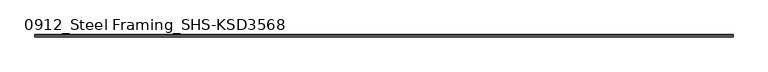
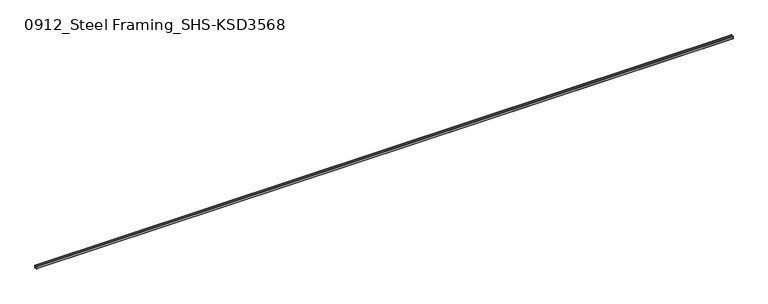
"""IFC4 building model written with IfcOpenShell, lengths in millimetres: beam geometry, 0912_Steel Framing_SHS-KSD3568 : H_SB_ASB_SHS-150x150x6."""

from ifc_helpers import new_model, si_unit, point, frame, frame_2d, origin, place, context, project, spatial, polyline, circle_curve, trimmed, segment, composite_curve, outline, extrude, source, transform, mapped, element, save


def beam_0912_steel_framing_shs_ksd3568_1b1479d8(model_context):
    return source(origin(), model_context, "Body", "SweptSolid", [
        extrude(outline(composite_curve([segment(polyline([(75.0, 63.0), (75.0, -63.0)]), True, "CONTINUOUS"), segment(trimmed(circle_curve(frame_2d((63.0, -63.0)), 12.0), [point((75.0, -63.0))], [point((63.0, -75.0))], False, "CARTESIAN"), True, "CONTINUOUS"), segment(polyline([(63.0, -75.0), (-63.0, -75.0)]), True, "CONTINUOUS"), segment(trimmed(circle_curve(frame_2d((-63.0, -63.0)), 12.0), [point((-63.0, -75.0))], [point((-75.0, -63.0))], False, "CARTESIAN"), True, "CONTINUOUS"), segment(polyline([(-75.0, -63.0), (-75.0, 63.0)]), True, "CONTINUOUS"), segment(trimmed(circle_curve(frame_2d((-63.0, 63.0)), 12.0), [point((-75.0, 63.0))], [point((-63.0, 75.0))], False, "CARTESIAN"), True, "CONTINUOUS"), segment(polyline([(-63.0, 75.0), (63.0, 75.0)]), True, "CONTINUOUS"), segment(trimmed(circle_curve(frame_2d((63.0, 63.0)), 12.0), [point((63.0, 75.0))], [point((75.0, 63.0))], False, "CARTESIAN"), True, "CONTINUOUS")], self_intersect=False), holes=[composite_curve([segment(trimmed(circle_curve(frame_2d((-63.0, 63.0)), 6.0), [point((-63.0, 69.0))], [point((-69.0, 63.0))], True, "CARTESIAN"), True, "CONTINUOUS"), segment(polyline([(-69.0, 63.0), (-69.0, -63.0)]), True, "CONTINUOUS"), segment(trimmed(circle_curve(frame_2d((-63.0, -63.0)), 6.0), [point((-69.0, -63.0))], [point((-63.0, -69.0))], True, "CARTESIAN"), True, "CONTINUOUS"), segment(polyline([(-63.0, -69.0), (63.0, -69.0)]), True, "CONTINUOUS"), segment(trimmed(circle_curve(frame_2d((63.0, -63.0)), 6.0), [point((63.0, -69.0))], [point((69.0, -63.0))], True, "CARTESIAN"), True, "CONTINUOUS"), segment(polyline([(69.0, -63.0), (69.0, 63.0)]), True, "CONTINUOUS"), segment(trimmed(circle_curve(frame_2d((63.0, 63.0)), 6.0), [point((69.0, 63.0))], [point((63.0, 69.0))], True, "CARTESIAN"), True, "CONTINUOUS"), segment(polyline([(63.0, 69.0), (-63.0, 69.0)]), True, "CONTINUOUS")], self_intersect=False)]), frame((-20590.0, 0.0, 0.0), z_axis=(1.0, 0.0, 0.0), x_axis=(0.0, 1.0, 0.0)), (0.0, 0.0, 1.0), 41180.0),
    ])


if __name__ == "__main__":
    model = new_model("IFC4")
    model_context = context("Model", 3, world=origin())
    ifc_project = project(units=[si_unit("LENGTHUNIT", "METRE", prefix="MILLI")], contexts=[model_context])
    site = spatial("IfcSite", under=ifc_project)
    building = spatial("IfcBuilding", under=site)
    placement = place(None, origin())
    beam_0912_steel_framing_shs_ksd3568_shape = beam_0912_steel_framing_shs_ksd3568_1b1479d8(model_context)
    element("IfcBeam", 1, ObjectType="0912_Steel Framing_SHS-KSD3568 : H_SB_ASB_SHS-150x150x6", at=placement, inside=building, context=model_context, shape_type="MappedRepresentation", body=[
        mapped(beam_0912_steel_framing_shs_ksd3568_shape, transform((0.0, 0.0, 0.0), x_axis=(1.0, 0.0, 0.0), y_axis=(0.0, 1.0, 0.0), z_axis=(0.0, 0.0, 1.0))),
    ])
    save(model, "model.ifc")

# Revit data of these elements
# Type "0912_Steel Framing_SHS-KSD3568 : H_SB_ASB_SHS-150x150x6"
#   H_WM Code_1 = "S01AA002-00001 | Main Steel Structure Fabrication Work | Shelter/Building | Medium Steel - Standard (90KG/M>Weight≥30KG/M) | Material: (   )"
#   H_WM Code_2 = "S03AA028-00001 | Main Steel Structure Erection Work | Shelter/Building | Medium Steel (90KG/M>Weight≥30KG/M) | Material: (   )"
#   H_WM Code_3 = "S01AA010-00001 | Main Steel Structure Fabrication Work | Shelter/Building | Steel Painting/Coating | for Non-Fireproofed Steel Surface, Surface Preparation, Primer, Second & Final Coat | Material: (   )"
#   H_Q'ty Cal Type Tag = "SB-Q2"
#   Perimeter = 0.60 m²/m
#   Nominal Weight = 26.40 kgf/m
#   Length [instance default] = 1.0000 m
#   b = 0.1500 m
#   h = 0.1500 m
#   tr = 0.0120 m
#   t = 0.0060 m
#   A = 28.36 m²
#   Structural Material [instance default] = Steel, 45-345
# Element 1 (IfcBeam, "0912_Steel Framing_SHS-KSD3568 : H_SB_ASB_SHS-150x150x6")
#   Structural Material = none
# Materials
#   "Steel, 45-345": class "Metal", colour RGB 189 187 185, transparency 0, Description = "Steel 345 MPa", Cost = 0
